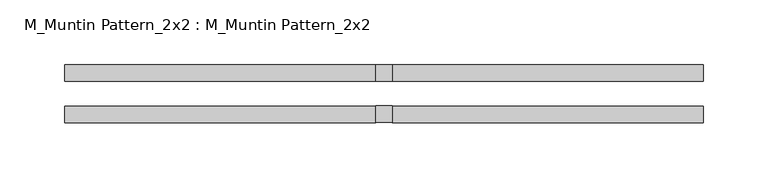
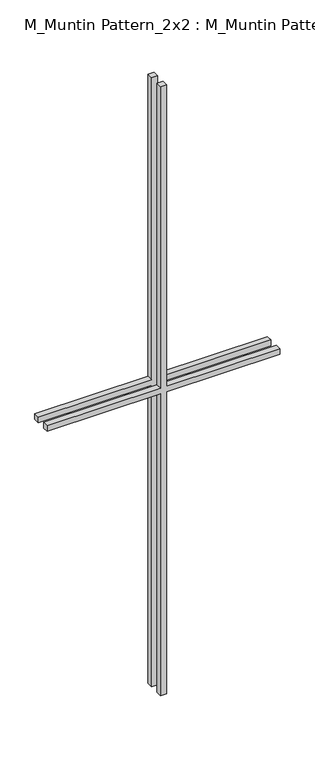
"""IFC4 building model written with IfcOpenShell, lengths in millimetres: proxy geometry, M_Muntin Pattern_2x2 : M_Muntin Pattern_2x2."""

from ifc_helpers import new_model, si_unit, frame, origin, place, context, project, spatial, polyline, outline, extrude, source, transform, mapped, element, save


def m_muntin_pattern_2x2_m_muntin_pattern_2x2_0b9f2fee(model_context):
    return source(origin(), model_context, "Body", "SweptSolid", [
        extrude(outline(polyline([(686.5, -6.35), (686.5, -246.1999152), (673.8, -246.1999152), (673.8, -6.35), (0.0, -6.35), (0.0, 6.35), (673.8, 6.35), (673.8, 246.1999152), (686.5, 246.1999152), (686.5, 6.35), (1360.3, 6.35), (1360.3, -6.35), (686.5, -6.35)])), frame((0.0, 9.525, 0.0), z_axis=(0.0, 1.0, 0.0), x_axis=(0.0, 0.0, 1.0)), (0.0, 0.0, 1.0), 12.7),
        extrude(outline(polyline([(686.5, -6.35), (686.5, -246.1999152), (673.8, -246.1999152), (673.8, -6.35), (0.0, -6.35), (0.0, 6.35), (673.8, 6.35), (673.8, 246.1999152), (686.5, 246.1999152), (686.5, 6.35), (1360.3, 6.35), (1360.3, -6.35), (686.5, -6.35)])), frame((0.0, -22.225, 0.0), z_axis=(0.0, 1.0, 0.0), x_axis=(0.0, 0.0, 1.0)), (0.0, 0.0, 1.0), 12.7),
    ])


if __name__ == "__main__":
    model = new_model("IFC4")
    model_context = context("Model", 3, world=origin())
    ifc_project = project(units=[si_unit("LENGTHUNIT", "METRE", prefix="MILLI")], contexts=[model_context])
    site = spatial("IfcSite", under=ifc_project)
    building = spatial("IfcBuilding", under=site)
    placement = place(None, origin())
    m_muntin_pattern_2x2_m_muntin_pattern_2x2_shape = m_muntin_pattern_2x2_m_muntin_pattern_2x2_0b9f2fee(model_context)
    element("IfcBuildingElementProxy", 1, Name="M_Muntin Pattern_2x2 : M_Muntin Pattern_2x2", ObjectType="M_Muntin Pattern_2x2 : M_Muntin Pattern_2x2", at=placement, inside=building, context=model_context, shape_type="MappedRepresentation", body=[
        mapped(m_muntin_pattern_2x2_m_muntin_pattern_2x2_shape, transform((0.0, 0.0, 0.0), x_axis=(1.0, 0.0, 0.0), y_axis=(0.0, 1.0, 0.0), z_axis=(0.0, 0.0, 1.0))),
    ])
    save(model, "model.ifc")

# Revit data of these elements
# Type "M_Muntin Pattern_2x2 : M_Muntin Pattern_2x2"
#   Width [instance default] = 1200 mm
#   Thickness = 12.7 mm
#   Height [instance default] = 1200 mm
#   Distance = 19.05 mm
#   Interior Material [instance default] = none
#   Exterior Material [instance default] = none
#   Default Elevation = 0
# Element 1 (IfcBuildingElementProxy, "M_Muntin Pattern_2x2 : M_Muntin Pattern_2x2")
#   Width = 492.4 mm
#   Height = 1360.3 mm
#   Interior Material = Wood - Stained
#   Exterior Material = Clad - White
#   Materials on its faces: "Clad - White", "Wood - Stained"
# Materials
#   "Clad - White": class "Wood", colour RGB 242 242 238, transparency 0, Cost = 0
#   "Wood - Stained": class "Wood", colour RGB 227 170 128, transparency 0, Cost = 0
